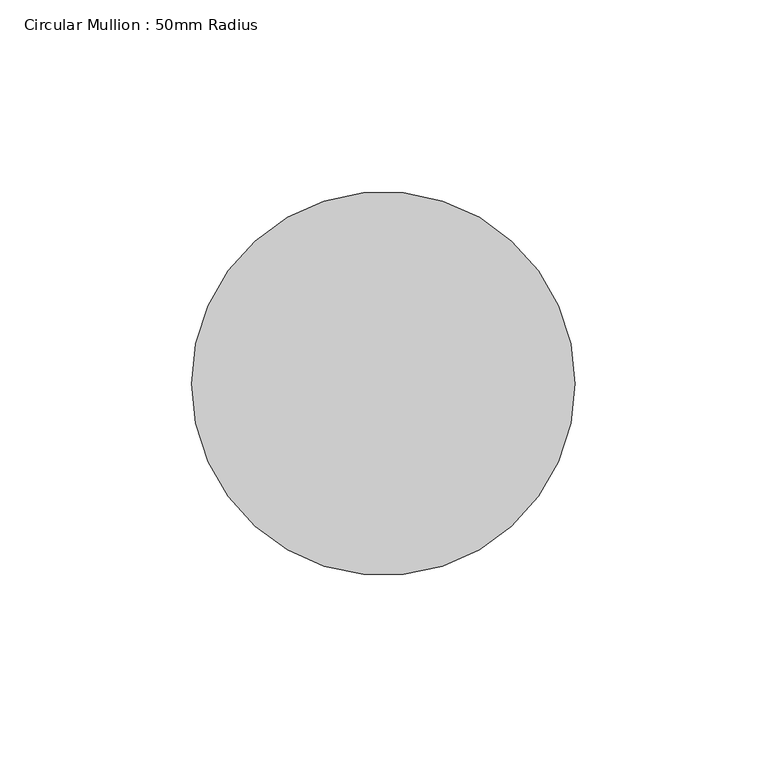
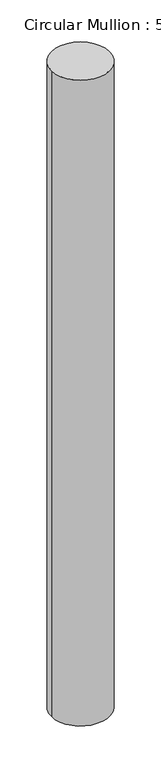
"""IFC4 building model written with IfcOpenShell, lengths in millimetres: member geometry, Circular Mullion : 50mm Radius."""

from ifc_helpers import new_model, si_unit, point, frame, origin, origin_2d, place, context, project, spatial, circle_curve, trimmed, segment, composite_curve, outline, extrude, source, transform, mapped, element, save


def circular_mullion_50mm_radius_64b3ba2e(model_context):
    return source(origin(), model_context, "Body", "SweptSolid", [
        extrude(outline(composite_curve([segment(trimmed(circle_curve(origin_2d(), 50.0), [point((50.0, 0.0))], [point((-50.0, 0.0))], False, "CARTESIAN"), True, "CONTINUOUS"), segment(trimmed(circle_curve(origin_2d(), 50.0), [point((-50.0, 0.0))], [point((50.0, 0.0))], False, "CARTESIAN"), True, "CONTINUOUS")], self_intersect=False)), frame((0.0, 0.0, -1176.1166401), z_axis=(0.0, 0.0, 1.0), x_axis=(1.0, 0.0, 0.0)), (0.0, 0.0, 1.0), 1176.1166401),
    ])


if __name__ == "__main__":
    model = new_model("IFC4")
    model_context = context("Model", 3, world=origin())
    ifc_project = project(units=[si_unit("LENGTHUNIT", "METRE", prefix="MILLI")], contexts=[model_context])
    site = spatial("IfcSite", under=ifc_project)
    building = spatial("IfcBuilding", under=site)
    placement = place(None, origin())
    circular_mullion_50mm_radius_shape = circular_mullion_50mm_radius_64b3ba2e(model_context)
    element("IfcMember", 1, ObjectType="Circular Mullion : 50mm Radius", at=placement, inside=building, context=model_context, shape_type="MappedRepresentation", body=[
        mapped(circular_mullion_50mm_radius_shape, transform((0.0, 0.0, 0.0), x_axis=(1.0, 0.0, 0.0), y_axis=(0.0, 1.0, 0.0), z_axis=(0.0, 0.0, 1.0))),
    ])
    save(model, "model.ifc")

# Revit data of these elements
# Type "Circular Mullion : 50mm Radius"
#   built-in parameter 1007350 = 0.164042 (stored number, unit not read)
# Element 1 (IfcMember, "Circular Mullion : 50mm Radius")
#   Materials on its faces: "Aluminium"
# Materials
#   "Aluminium": class "Metal", colour RGB 247 247 247, transparency 0, Description = "Aluminium 6061", Cost = 0
